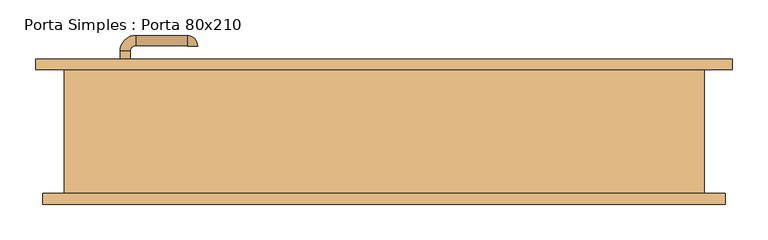
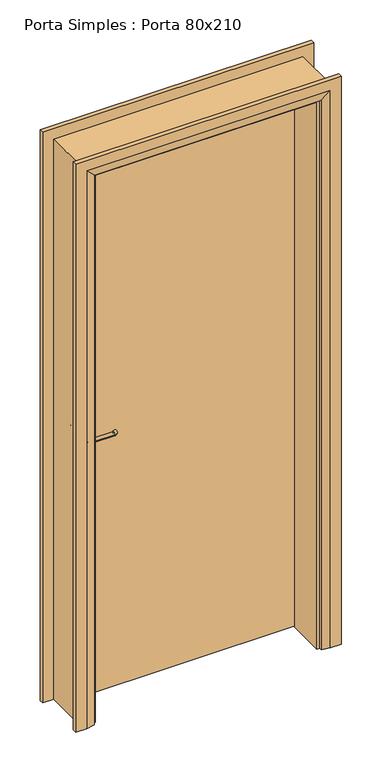
"""IFC4 building model written with IfcOpenShell, lengths in millimetres: door geometry, Porta Simples : Porta 80x210."""

from ifc_helpers import new_model, si_unit, point, frame, frame_2d, origin, place, context, project, spatial, polyline, circle_curve, ellipse_curve, trimmed, segment, composite_curve, outline, extrude, faceted_brep, source, transform, mapped, element, save
from ifc_brep_helpers import plane_surface, cylinder_surface, revolved_surface, advanced_brep


def porta_simples_porta_80x210_892b00d0(model_context):
    return source(origin(), model_context, "Body", "SolidModel", [
        extrude(outline(composite_curve([segment(trimmed(circle_curve(frame_2d((1050.0, -364.0)), 20.0), [point((1050.0, -384.0))], [point((1050.0, -344.0))], False, "CARTESIAN"), True, "CONTINUOUS"), segment(trimmed(circle_curve(frame_2d((1050.0, -364.0)), 20.0), [point((1050.0, -344.0))], [point((1050.0, -384.0))], False, "CARTESIAN"), True, "CONTINUOUS")], self_intersect=False)), frame((0.0, 41.7070105, 0.0), z_axis=(0.0, 1.0, 0.0), x_axis=(0.0, 0.0, 1.0)), (0.0, 0.0, 1.0), 4.5929895),
        advanced_brep(
        [(-357.0, 41.7070105, 1050.0), (-371.0, 41.7070105, 1050.0), (-371.0, 26.3, 1050.0), (-357.0, 26.3, 1050.0), (-349.0, 4.3, 1050.0), (-349.0, 18.3, 1050.0), (-277.0, 4.3, 1050.0), (-277.0, 18.3, 1050.0), (-276.0, 19.3, 1050.0), (-262.0, 19.3, 1050.0)],
        [
            (0, 1, circle_curve(frame((-364.0, 41.7070105, 1050.0), z_axis=(0.0, 1.0, 0.0), x_axis=(-1.0, 0.0, 0.0)), 7.0)),
            (1, 0, circle_curve(frame((-364.0, 41.7070105, 1050.0), z_axis=(0.0, 1.0, 0.0), x_axis=(-1.0, 0.0, 0.0)), 7.0)),
            (1, 2),
            (2, 3, circle_curve(frame((-364.0, 26.3, 1050.0), z_axis=(0.0, 1.0, 0.0), x_axis=(-1.0, 0.0, 0.0)), 7.0)),
            (3, 0),
            (3, 2, circle_curve(frame((-364.0, 26.3, 1050.0), z_axis=(0.0, 1.0, 0.0), x_axis=(-1.0, 0.0, 0.0)), 7.0)),
            (4, 5, circle_curve(frame((-349.0, 11.3, 1050.0), z_axis=(-1.0, 0.0, 0.0), x_axis=(0.0, -1.0, 0.0)), 7.0)),
            (5, 3, circle_curve(frame((-349.0, 26.3, 1050.0), z_axis=(0.0, 0.0, -1.0), x_axis=(-1.0, 0.0, 0.0)), 8.0)),
            (2, 4, circle_curve(frame((-349.0, 26.3, 1050.0), z_axis=(0.0, 0.0, 1.0), x_axis=(-1.0, 0.0, 0.0)), 22.0)),
            (5, 4, circle_curve(frame((-349.0, 11.3, 1050.0), z_axis=(-1.0, 0.0, 0.0), x_axis=(0.0, -1.0, 0.0)), 7.0)),
            (4, 6),
            (6, 7, circle_curve(frame((-277.0, 11.3, 1050.0), z_axis=(-1.0, 0.0, 0.0), x_axis=(0.0, -1.0, 0.0)), 7.0)),
            (7, 5),
            (7, 6, circle_curve(frame((-277.0, 11.3, 1050.0), z_axis=(-1.0, 0.0, 0.0), x_axis=(0.0, -1.0, 0.0)), 7.0)),
            (8, 9, circle_curve(frame((-269.0, 19.3, 1050.0), z_axis=(0.0, 1.0, 0.0), x_axis=(1.0, 0.0, 0.0)), 7.0)),
            (9, 8, circle_curve(frame((-269.0, 19.3, 1050.0), z_axis=(0.0, 1.0, 0.0), x_axis=(1.0, 0.0, 0.0)), 7.0)),
            (8, 7, circle_curve(frame((-277.0, 19.3, 1050.0), z_axis=(0.0, 0.0, -1.0), x_axis=(0.0, -1.0, 0.0)), 1.0)),
            (6, 9, circle_curve(frame((-277.0, 19.3, 1050.0), z_axis=(0.0, 0.0, 1.0), x_axis=(0.0, -1.0, 0.0)), 15.0)),
        ],
        [
            plane_surface(frame((-364.0, 41.7070105, 1050.0), z_axis=(0.0, 1.0, 0.0), x_axis=(0.0, 0.0, 1.0))),
            cylinder_surface(frame((-364.0, 41.7070105, 1050.0), z_axis=(0.0, 1.0, 0.0), x_axis=(-1.0, 0.0, 0.0)), 7.0),
            revolved_surface(trimmed(ellipse_curve(frame((-364.0, 26.3, 1050.0), z_axis=(0.0, -1.0, 0.0), x_axis=(-1.0, 0.0, 0.0)), 7.0, 7.0), [point((-357.0, 26.3, 1050.0))], [point((-371.0, 26.3, 1050.0))], True, "CARTESIAN"), (-349.0, 26.3, 1050.0), (0.0, 0.0, -1.0)),
            revolved_surface(trimmed(ellipse_curve(frame((-364.0, 26.3, 1050.0), z_axis=(0.0, -1.0, 0.0), x_axis=(-1.0, 0.0, 0.0)), 7.0, 7.0), [point((-371.0, 26.3, 1050.0))], [point((-357.0, 26.3, 1050.0))], True, "CARTESIAN"), (-349.0, 26.3, 1050.0), (0.0, 0.0, -1.0)),
            cylinder_surface(frame((-349.0, 11.3, 1050.0), z_axis=(-1.0, 0.0, 0.0), x_axis=(0.0, -1.0, 0.0)), 7.0),
            plane_surface(frame((-269.0, 19.3, 1050.0), z_axis=(0.0, 1.0, 0.0), x_axis=(0.0, 0.0, 1.0))),
            revolved_surface(trimmed(ellipse_curve(frame((-277.0, 11.3, 1050.0), z_axis=(1.0, 0.0, 0.0), x_axis=(0.0, -1.0, 0.0)), 7.0, 7.0), [point((-277.0, 18.3, 1050.0))], [point((-277.0, 4.3, 1050.0))], True, "CARTESIAN"), (-277.0, 19.3, 1050.0), (0.0, 0.0, -1.0)),
            revolved_surface(trimmed(ellipse_curve(frame((-277.0, 11.3, 1050.0), z_axis=(1.0, 0.0, 0.0), x_axis=(0.0, -1.0, 0.0)), 7.0, 7.0), [point((-277.0, 4.3, 1050.0))], [point((-277.0, 18.3, 1050.0))], True, "CARTESIAN"), (-277.0, 19.3, 1050.0), (0.0, 0.0, -1.0)),
        ],
        [
            (0, [[1, 2]]),
            (1, [[3, 4, 5, -2]]),
            (1, [[-5, 6, -3, -1]]),
            (2, [[7, 8, -4, 9]]),
            (3, [[10, -9, -6, -8]]),
            (4, [[11, 12, 13, -7]]),
            (4, [[-13, 14, -11, -10]]),
            (5, [[15, 16]]),
            (6, [[-15, 17, -12, 18]]),
            (7, [[-16, -18, -14, -17]]),
        ],
    ),
        extrude(outline(polyline([(-334.0, 52.3), (-334.0, 46.3), (-394.0, 46.3), (-394.0, 52.3), (-334.0, 52.3)])), frame((0.0, 0.0, 925.0), z_axis=(0.0, 0.0, 1.0), x_axis=(1.0, 0.0, 0.0)), (0.0, 0.0, 1.0), 165.0),
        extrude(outline(composite_curve([segment(trimmed(circle_curve(frame_2d((1050.0, -364.0)), 20.0), [point((1050.0, -384.0))], [point((1050.0, -344.0))], False, "CARTESIAN"), True, "CONTINUOUS"), segment(trimmed(circle_curve(frame_2d((1050.0, -364.0)), 20.0), [point((1050.0, -344.0))], [point((1050.0, -384.0))], False, "CARTESIAN"), True, "CONTINUOUS")], self_intersect=False)), frame((0.0, 93.3, 0.0), z_axis=(0.0, 1.0, 0.0), x_axis=(0.0, 0.0, 1.0)), (0.0, 0.0, 1.0), 4.5929895),
        advanced_brep(
        [(-357.0, 97.8929895, 1050.0), (-371.0, 97.8929895, 1050.0), (-357.0, 113.3, 1050.0), (-371.0, 113.3, 1050.0), (-349.0, 135.3, 1050.0), (-349.0, 121.3, 1050.0), (-277.0, 121.3, 1050.0), (-277.0, 135.3, 1050.0), (-276.0, 120.3, 1050.0), (-262.0, 120.3, 1050.0)],
        [
            (0, 1, circle_curve(frame((-364.0, 97.8929895, 1050.0), z_axis=(0.0, -1.0, 0.0), x_axis=(-1.0, 0.0, 0.0)), 7.0)),
            (1, 0, circle_curve(frame((-364.0, 97.8929895, 1050.0), z_axis=(0.0, -1.0, 0.0), x_axis=(-1.0, 0.0, 0.0)), 7.0)),
            (0, 2),
            (2, 3, circle_curve(frame((-364.0, 113.3, 1050.0), z_axis=(0.0, -1.0, 0.0), x_axis=(-1.0, 0.0, 0.0)), 7.0)),
            (3, 1),
            (3, 2, circle_curve(frame((-364.0, 113.3, 1050.0), z_axis=(0.0, -1.0, 0.0), x_axis=(-1.0, 0.0, 0.0)), 7.0)),
            (4, 3, circle_curve(frame((-349.0, 113.3, 1050.0), z_axis=(0.0, 0.0, 1.0), x_axis=(-1.0, 0.0, 0.0)), 22.0)),
            (2, 5, circle_curve(frame((-349.0, 113.3, 1050.0), z_axis=(0.0, 0.0, -1.0), x_axis=(-1.0, 0.0, 0.0)), 8.0)),
            (5, 4, circle_curve(frame((-349.0, 128.3, 1050.0), z_axis=(-1.0, 0.0, 0.0), x_axis=(0.0, 1.0, 0.0)), 7.0)),
            (4, 5, circle_curve(frame((-349.0, 128.3, 1050.0), z_axis=(-1.0, 0.0, 0.0), x_axis=(0.0, 1.0, 0.0)), 7.0)),
            (5, 6),
            (6, 7, circle_curve(frame((-277.0, 128.3, 1050.0), z_axis=(-1.0, 0.0, 0.0), x_axis=(0.0, 1.0, 0.0)), 7.0)),
            (7, 4),
            (7, 6, circle_curve(frame((-277.0, 128.3, 1050.0), z_axis=(-1.0, 0.0, 0.0), x_axis=(0.0, 1.0, 0.0)), 7.0)),
            (8, 9, circle_curve(frame((-269.0, 120.3, 1050.0), z_axis=(0.0, -1.0, 0.0), x_axis=(1.0, 0.0, 0.0)), 7.0)),
            (9, 8, circle_curve(frame((-269.0, 120.3, 1050.0), z_axis=(0.0, -1.0, 0.0), x_axis=(1.0, 0.0, 0.0)), 7.0)),
            (9, 7, circle_curve(frame((-277.0, 120.3, 1050.0), z_axis=(0.0, 0.0, 1.0), x_axis=(0.0, 1.0, 0.0)), 15.0)),
            (6, 8, circle_curve(frame((-277.0, 120.3, 1050.0), z_axis=(0.0, 0.0, -1.0), x_axis=(0.0, 1.0, 0.0)), 1.0)),
        ],
        [
            plane_surface(frame((-364.0, 97.8929895, 1050.0), z_axis=(0.0, -1.0, 0.0), x_axis=(0.0, 0.0, 1.0))),
            cylinder_surface(frame((-364.0, 97.8929895, 1050.0), z_axis=(0.0, -1.0, 0.0), x_axis=(-1.0, 0.0, 0.0)), 7.0),
            revolved_surface(trimmed(ellipse_curve(frame((-364.0, 113.3, 1050.0), z_axis=(0.0, -1.0, 0.0), x_axis=(-1.0, 0.0, 0.0)), 7.0, 7.0), [point((-357.0, 113.3, 1050.0))], [point((-371.0, 113.3, 1050.0))], True, "CARTESIAN"), (-349.0, 113.3, 1050.0), (0.0, 0.0, -1.0)),
            revolved_surface(trimmed(ellipse_curve(frame((-364.0, 113.3, 1050.0), z_axis=(0.0, -1.0, 0.0), x_axis=(-1.0, 0.0, 0.0)), 7.0, 7.0), [point((-371.0, 113.3, 1050.0))], [point((-357.0, 113.3, 1050.0))], True, "CARTESIAN"), (-349.0, 113.3, 1050.0), (0.0, 0.0, -1.0)),
            cylinder_surface(frame((-349.0, 128.3, 1050.0), z_axis=(-1.0, 0.0, 0.0), x_axis=(0.0, 1.0, 0.0)), 7.0),
            plane_surface(frame((-269.0, 120.3, 1050.0), z_axis=(0.0, -1.0, 0.0), x_axis=(0.0, 0.0, 1.0))),
            revolved_surface(trimmed(ellipse_curve(frame((-277.0, 128.3, 1050.0), z_axis=(-1.0, 0.0, 0.0), x_axis=(0.0, 1.0, 0.0)), 7.0, 7.0), [point((-277.0, 121.3, 1050.0))], [point((-277.0, 135.3, 1050.0))], True, "CARTESIAN"), (-277.0, 120.3, 1050.0), (0.0, 0.0, -1.0)),
            revolved_surface(trimmed(ellipse_curve(frame((-277.0, 128.3, 1050.0), z_axis=(-1.0, 0.0, 0.0), x_axis=(0.0, 1.0, 0.0)), 7.0, 7.0), [point((-277.0, 135.3, 1050.0))], [point((-277.0, 121.3, 1050.0))], True, "CARTESIAN"), (-277.0, 120.3, 1050.0), (0.0, 0.0, -1.0)),
        ],
        [
            (0, [[1, 2]]),
            (1, [[-1, 3, 4, 5]]),
            (1, [[-2, -5, 6, -3]]),
            (2, [[7, -4, 8, 9]]),
            (3, [[-8, -6, -7, 10]]),
            (4, [[-9, 11, 12, 13]]),
            (4, [[-10, -13, 14, -11]]),
            (5, [[15, 16]]),
            (6, [[17, -12, 18, -16]]),
            (7, [[-18, -14, -17, -15]]),
        ],
    ),
        extrude(outline(polyline([(-334.0, 87.3), (-394.0, 87.3), (-394.0, 93.3), (-334.0, 93.3), (-334.0, 87.3)])), frame((0.0, 0.0, 925.0), z_axis=(0.0, 0.0, 1.0), x_axis=(1.0, 0.0, 0.0)), (0.0, 0.0, 1.0), 165.0),
        extrude(outline(polyline([(408.0, 52.3), (-408.0, 52.3), (-408.0, 87.3), (408.0, 87.3), (408.0, 52.3)])), frame((0.0, 0.0, 53.0), z_axis=(0.0, 0.0, 1.0), x_axis=(1.0, 0.0, 0.0)), (0.0, 0.0, 1.0), 2094.0),
        faceted_brep([(480.0, -87.3, 50.0), (480.0, -102.3, 50.0), (440.0, -102.3, 50.0), (410.0, -97.3, 50.0), (410.0, -87.3, 50.0), (480.0, -87.3, 2220.0), (480.0, -102.3, 2220.0), (-480.0, -102.3, 2220.0), (-480.0, -102.3, 50.0), (-440.0, -102.3, 50.0), (-440.0, -102.3, 2180.0), (440.0, -102.3, 2180.0), (410.0, -97.3, 2150.0), (410.0, -87.3, 2150.0), (-410.0, -87.3, 2150.0), (-410.0, -87.3, 50.0), (-480.0, -87.3, 50.0), (-480.0, -87.3, 2220.0), (-410.0, -97.3, 2150.0), (-410.0, -97.3, 50.0)], [[[0, 1, 2, 3, 4]], [[1, 0, 5, 6]], [[2, 1, 6, 7, 8, 9, 10, 11]], [[3, 2, 11, 12]], [[4, 3, 12, 13]], [[0, 4, 13, 14, 15, 16, 17, 5]], [[14, 18, 19, 15]], [[16, 15, 19, 9, 8]], [[7, 17, 16, 8]], [[18, 10, 9, 19]], [[13, 12, 18, 14]], [[6, 5, 17, 7]], [[12, 11, 10, 18]]]),
        faceted_brep([(490.0, 87.3, 50.0), (420.0, 87.3, 50.0), (420.0, 97.3, 50.0), (450.0, 102.3, 50.0), (490.0, 102.3, 50.0), (490.0, 87.3, 2230.0), (-490.0, 87.3, 2230.0), (-490.0, 87.3, 50.0), (-420.0, 87.3, 50.0), (-420.0, 87.3, 2160.0), (420.0, 87.3, 2160.0), (420.0, 97.3, 2160.0), (450.0, 102.3, 2190.0), (-450.0, 102.3, 2190.0), (-450.0, 102.3, 50.0), (-490.0, 102.3, 50.0), (-490.0, 102.3, 2230.0), (490.0, 102.3, 2230.0), (-420.0, 97.3, 50.0), (-420.0, 97.3, 2160.0)], [[[0, 1, 2, 3, 4]], [[1, 0, 5, 6, 7, 8, 9, 10]], [[2, 1, 10, 11]], [[3, 2, 11, 12]], [[4, 3, 12, 13, 14, 15, 16, 17]], [[0, 4, 17, 5]], [[6, 16, 15, 7]], [[7, 15, 14, 18, 8]], [[19, 9, 8, 18]], [[13, 19, 18, 14]], [[11, 10, 9, 19]], [[5, 17, 16, 6]], [[12, 11, 19, 13]]]),
        faceted_brep([(-410.0, 87.3, 50.0), (-410.0, 50.3, 50.0), (-400.0, 50.3, 50.0), (-400.0, -87.3, 50.0), (-450.0, -87.3, 50.0), (-450.0, 87.3, 50.0), (-410.0, 87.3, 2150.0), (-410.0, 50.3, 2150.0), (-400.0, 50.3, 2140.0), (-400.0, -87.3, 2140.0), (-450.0, -87.3, 2190.0), (-450.0, 87.3, 2190.0), (410.0, 87.3, 50.0), (450.0, 87.3, 50.0), (450.0, -87.3, 50.0), (400.0, -87.3, 50.0), (400.0, 50.3, 50.0), (410.0, 50.3, 50.0), (410.0, 87.3, 2150.0), (450.0, 87.3, 2190.0), (450.0, -87.3, 2190.0), (400.0, -87.3, 2140.0), (400.0, 50.3, 2140.0), (410.0, 50.3, 2150.0)], [[[0, 1, 2, 3, 4, 5]], [[1, 0, 6, 7]], [[2, 1, 7, 8]], [[3, 2, 8, 9]], [[4, 3, 9, 10]], [[5, 4, 10, 11]], [[0, 5, 11, 6]], [[12, 13, 14, 15, 16, 17]], [[18, 19, 13, 12]], [[19, 20, 14, 13]], [[20, 21, 15, 14]], [[21, 22, 16, 15]], [[22, 23, 17, 16]], [[23, 18, 12, 17]], [[7, 6, 18, 23]], [[8, 7, 23, 22]], [[9, 8, 22, 21]], [[10, 9, 21, 20]], [[11, 10, 20, 19]], [[6, 11, 19, 18]]]),
    ])


if __name__ == "__main__":
    model = new_model("IFC4")
    model_context = context("Model", 3, world=origin())
    ifc_project = project(units=[si_unit("LENGTHUNIT", "METRE", prefix="MILLI")], contexts=[model_context])
    site = spatial("IfcSite", under=ifc_project)
    building = spatial("IfcBuilding", under=site)
    placement = place(None, origin())
    porta_simples_porta_80x210_shape = porta_simples_porta_80x210_892b00d0(model_context)
    element("IfcDoor", 1, ObjectType="Porta Simples : Porta 80x210", at=placement, inside=building, context=model_context, shape_type="MappedRepresentation", body=[
        mapped(porta_simples_porta_80x210_shape, transform((0.0, 0.0, 0.0), x_axis=(1.0, 0.0, 0.0), y_axis=(0.0, 1.0, 0.0), z_axis=(0.0, 0.0, 1.0))),
    ])
    save(model, "model.ifc")

# Revit data of these elements
# Type "Porta Simples : Porta 80x210"
#   Type Mark = "49"
#   SINAPI = ""
#   Analytic Construction = "<Nenhum>"
#   Construction Type = "300"
#   Maçaneta [instance default] = ""
#   Fechadura [instance default] = ""
#   Vão Luz (somente para informação) = 0.78 m
#   Tolerância Folha Vertical = 0.003 m
#   Módulo Básico M = 0.10 m
#   Largura de Coordenação Modular Largura CM = 0.90 m
#   Rough Width = 0.90 m
#   Deslocamento da Horizontal da Folha = 0.00 m
#   Altura de Coordenação Modular Largura CM = 2.20 m
#   Rough Height = 2.20 m
#   Altura Nominal = 2.09 m
#   Ajuste de Coordenação Topo AC Topo = 0.01 m
#   Ajuste de Coordenação Base AC Base = 0.05 m
#   Ajuste de Coordenação AC = 0.01 m
#   Tolerância Folha Horizontal = 0.002 m
#   Largura Folha (somente para informação) = 0.796 m
#   Espessura Folha = 0.035 m
#   Maçaneta - Distância da Folha = 0.044 m
#   Maçaneta - Altura = 1.00 m
#   Largura Nominal (Largura Mn) = 0.82 m
#   Distância do Nível = 0.003 m
#   Aduela Interna Espessura = 0.04 m
#   Aduela Externa Espessura = 0.05 m
#   Altura Folha (somente para informação) = 2.075 m
#   Height = 2.14 m
#   Width = 0.88 m
#   Número de Módulos Básicos nM Largura = 9
#   Número de Módulos Básicos nM Altura = 22
#   Marco Metálico = no
#   Aduela de Madeira = no
#   Aduela Metálica de Canto = no
#   Guarnição Reta = no
#   Guarnição Chanfrada = yes
#   Batente - Material [instance default] = none
#   Painel - Material [instance default] = none
#   Model = ""
#   Function = (empty or 0)
#   Description = (empty or 0)
#   Wall Closure = (empty or 0)
#   Assembly Code = ""
# Element 1 (IfcDoor, "Porta Simples : Porta 80x210")
#   Materials on its faces: "Porta - Maçaneta"
# Materials
#   "Porta - Maçaneta": class "Diversos", colour RGB 0 0 0, transparency 0
